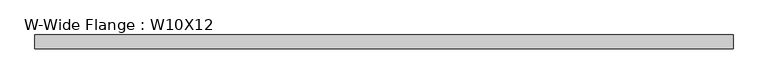
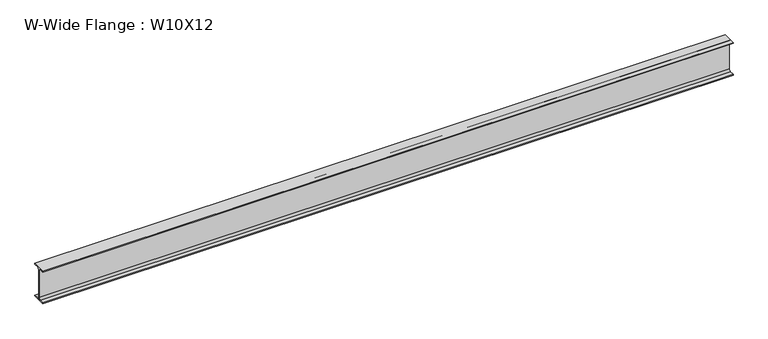
"""IFC4 building model written with IfcOpenShell, lengths in millimetres: beam geometry, W-Wide Flange : W10X12."""

from ifc_helpers import new_model, si_unit, point, frame, frame_2d, origin, place, context, project, spatial, polyline, circle_curve, trimmed, segment, composite_curve, outline, extrude, source, transform, mapped, element, save


def w_wide_flange_w10x12_2b4455fd(model_context):
    return source(origin(), model_context, "Body", "SweptSolid", [
        extrude(outline(composite_curve([segment(polyline([(50.292, -120.015), (50.292, -125.349), (-50.292, -125.349), (-50.292, -120.015), (-16.129, -120.015)]), True, "CONTINUOUS"), segment(trimmed(circle_curve(frame_2d((-16.129, -106.299)), 13.716), [point((-16.129, -120.015))], [point((-2.413, -106.299))], True, "CARTESIAN"), True, "CONTINUOUS"), segment(polyline([(-2.413, -106.299), (-2.413, 106.299)]), True, "CONTINUOUS"), segment(trimmed(circle_curve(frame_2d((-16.129, 106.299)), 13.716), [point((-2.413, 106.299))], [point((-16.129, 120.015))], True, "CARTESIAN"), True, "CONTINUOUS"), segment(polyline([(-16.129, 120.015), (-50.292, 120.015), (-50.292, 125.349), (50.292, 125.349), (50.292, 120.015), (16.129, 120.015)]), True, "CONTINUOUS"), segment(trimmed(circle_curve(frame_2d((16.129, 106.299)), 13.716), [point((16.129, 120.015))], [point((2.413, 106.299))], True, "CARTESIAN"), True, "CONTINUOUS"), segment(polyline([(2.413, 106.299), (2.413, -106.299)]), True, "CONTINUOUS"), segment(trimmed(circle_curve(frame_2d((16.129, -106.299)), 13.716), [point((2.413, -106.299))], [point((16.129, -120.015))], True, "CARTESIAN"), True, "CONTINUOUS"), segment(polyline([(16.129, -120.015), (50.292, -120.015)]), True, "CONTINUOUS")], self_intersect=False)), frame((-2535.2375, 0.0, 0.0), z_axis=(1.0, 0.0, 0.0), x_axis=(0.0, 1.0, 0.0)), (0.0, 0.0, 1.0), 5070.475),
    ])


if __name__ == "__main__":
    model = new_model("IFC4")
    model_context = context("Model", 3, world=origin())
    ifc_project = project(units=[si_unit("LENGTHUNIT", "METRE", prefix="MILLI")], contexts=[model_context])
    site = spatial("IfcSite", under=ifc_project)
    building = spatial("IfcBuilding", under=site)
    placement = place(None, origin())
    w_wide_flange_w10x12_shape = w_wide_flange_w10x12_2b4455fd(model_context)
    element("IfcBeam", 1, ObjectType="W-Wide Flange : W10X12", at=placement, inside=building, context=model_context, shape_type="MappedRepresentation", body=[
        mapped(w_wide_flange_w10x12_shape, transform((0.0, 0.0, 0.0), x_axis=(1.0, 0.0, 0.0), y_axis=(0.0, 1.0, 0.0), z_axis=(0.0, 0.0, 1.0))),
    ])
    save(model, "model.ifc")

# Revit data of these elements
# Type "W-Wide Flange : W10X12"
#   Assembly Code = "B10"
#   W = 12
#   Length [instance default] = 1524 mm
#   bf = 100.584 mm
#   d = 250.698 mm
#   k = 19.05 mm
#   k2 = 13.716 mm
#   tf = 5.334 mm
#   tw = 4.826 mm
#   A = 0.00228387 m²
#   Structural Material [instance default] = Steel ASTM A992
# Element 1 (IfcBeam, "W-Wide Flange : W10X12")
#   Structural Material = Aluminum, Anodized Red
#   Materials on its faces: "Aluminum, Anodized Red"
# Materials
#   "Steel ASTM A992": class "Metal", colour RGB 128 0 0, transparency 0, Description = "Structural steel 50ksi", Cost = 0
#   "Aluminum, Anodized Red": class "Metal", colour RGB 120 120 120, transparency 0, Description = "Anodized aluminum, red", Cost = 0
